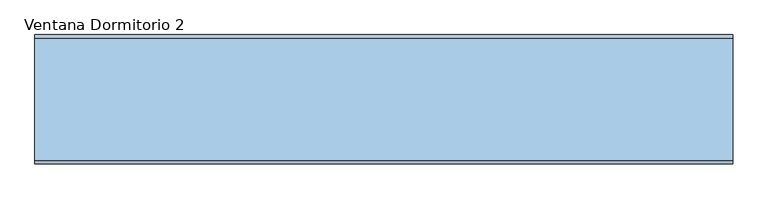
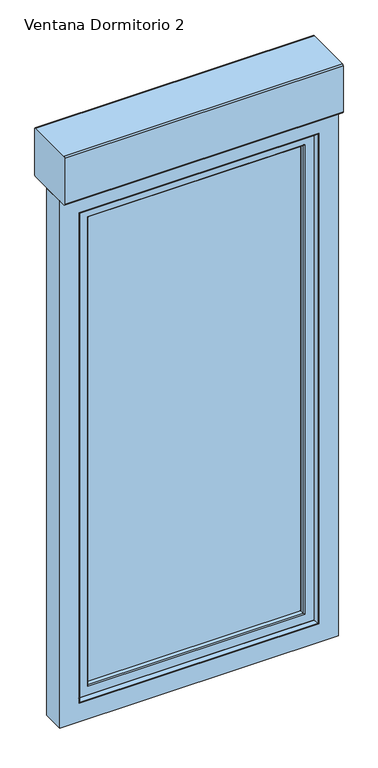
"""IFC4 building model written with IfcOpenShell, lengths in millimetres: window geometry, 2019_ES_Ventana_Replus_re80pvc301_10100_box_1-Hoja_con-Compacto : Ventana Dormitorio 2."""

import ifcopenshell
import ifcopenshell.guid

model = None  # the IFC model being written
_history = None  # IfcOwnerHistory: only IFC2X3 demands one
_inside = {}  # id of a spatial element -> (the spatial element, [elements in it])
_under = {}  # id of a project, library or spatial element -> (it, [spatial elements below it])
_declared = {}  # id of a project -> (the project, [libraries it declares])
_typed = {}  # id of a type object -> (the type object, [elements of that type])
_made_of = {}  # id of a material, layer set ... -> (it, [elements and type objects made of it])


def new_model(schema):
    """Start an empty IFC model of exactly this schema.

    Asked for "IFC4X3", IfcOpenShell would pick the latest addendum, in which some entities
    have other attributes; the version numbers below select the first issue.
    IFC2X3 requires an IfcOwnerHistory on every rooted entity: one is made here for all.
    """
    global model, _history
    if schema == "IFC4X3":
        model = ifcopenshell.file(schema_version=(4, 3, 0, 0))
    else:
        model = ifcopenshell.file(schema=schema)
    _inside.clear()
    _under.clear()
    _declared.clear()
    _typed.clear()
    _made_of.clear()
    _history = None
    if model.schema == "IFC2X3":
        org = make("IfcOrganization", Name="unknown")
        user = make(
            "IfcPersonAndOrganization",
            ThePerson=make("IfcPerson", FamilyName="unknown"),
            TheOrganization=org,
        )
        app = make(
            "IfcApplication",
            ApplicationDeveloper=org,
            Version="unknown",
            ApplicationFullName="unknown",
            ApplicationIdentifier="unknown",
        )
        _history = make(
            "IfcOwnerHistory",
            OwningUser=user,
            OwningApplication=app,
            ChangeAction="ADDED",
            CreationDate=0,
        )
    return model


def make(cls, **values):
    """One entity of the class cls with the attributes given. An attribute that is None is left unset."""
    return model.create_entity(
        cls, **{name: value for name, value in values.items() if value is not None}
    )


def rooted(cls, **values):
    """An entity with a GlobalId (a new one), such as an element, a storey or a relation."""
    return make(cls, GlobalId=ifcopenshell.guid.new(), OwnerHistory=_history, **values)


def si_unit(unit_type, name, prefix=None):
    """IfcSIUnit, for example si_unit("LENGTHUNIT", "METRE", prefix="MILLI")."""
    return make("IfcSIUnit", UnitType=unit_type, Prefix=prefix, Name=name)


def assignment(units):
    """IfcUnitAssignment: the units of a project."""
    return None if units is None else make("IfcUnitAssignment", Units=units)


def point(xyz):
    """IfcCartesianPoint."""
    return None if xyz is None else make("IfcCartesianPoint", Coordinates=xyz)


def direction(xyz):
    """IfcDirection."""
    return None if xyz is None else make("IfcDirection", DirectionRatios=xyz)


def frame(location, z_axis=None, x_axis=None):
    """IfcAxis2Placement3D, a coordinate frame: its origin and axes. An axis left out is left unset."""
    return make(
        "IfcAxis2Placement3D",
        Location=point(location),
        Axis=direction(z_axis),
        RefDirection=direction(x_axis),
    )


def frame_2d(location, x_axis=None):
    """IfcAxis2Placement2D, a coordinate frame in the plane: its origin and x axis."""
    return make(
        "IfcAxis2Placement2D", Location=point(location), RefDirection=direction(x_axis)
    )


def origin():
    """The frame at (0, 0, 0) with its axes left unset."""
    return frame((0.0, 0.0, 0.0))


def place(relative_to, where):
    """IfcLocalPlacement: puts the frame where relative to a parent placement (None: the world)."""
    return make(
        "IfcLocalPlacement", PlacementRelTo=relative_to, RelativePlacement=where
    )


def context(
    kind, dimensions, precision=None, world=None, true_north=None, identifier=None
):
    """IfcGeometricRepresentationContext, for example the 3D "Model" context."""
    return make(
        "IfcGeometricRepresentationContext",
        ContextIdentifier=identifier,
        ContextType=kind,
        CoordinateSpaceDimension=dimensions,
        Precision=precision,
        WorldCoordinateSystem=world,
        TrueNorth=true_north,
    )


def project(units=None, contexts=None):
    """IfcProject with its units and contexts."""
    return rooted(
        "IfcProject",
        Name="project",
        RepresentationContexts=contexts,
        UnitsInContext=assignment(units),
    )


def spatial(cls, under=None, at=None, **own):
    """A site, building, storey or space (cls), placed at a placement, below another one or the project."""
    s = rooted(cls, ObjectPlacement=at, **own)
    if under is not None:
        _under.setdefault(under.id(), (under, []))[1].append(s)
    return s


def polyline(points):
    """IfcPolyline through the points."""
    return make("IfcPolyline", Points=[point(p) for p in points])


def circle_curve(where, radius):
    """IfcCircle in the frame where."""
    return make("IfcCircle", Position=where, Radius=radius)


def ellipse_curve(where, semi_axis1, semi_axis2):
    """IfcEllipse in the frame where."""
    return make(
        "IfcEllipse", Position=where, SemiAxis1=semi_axis1, SemiAxis2=semi_axis2
    )


def trimmed(basis, trim1, trim2, sense, master):
    """IfcTrimmedCurve: the piece of a basis curve between two trims."""
    return make(
        "IfcTrimmedCurve",
        BasisCurve=basis,
        Trim1=trim1,
        Trim2=trim2,
        SenseAgreement=sense,
        MasterRepresentation=master,
    )


def segment(curve, same_sense, transition):
    """IfcCompositeCurveSegment."""
    return make(
        "IfcCompositeCurveSegment",
        Transition=transition,
        SameSense=same_sense,
        ParentCurve=curve,
    )


def composite_curve(segments, self_intersect=None):
    """IfcCompositeCurve: segments joined end to end."""
    return make("IfcCompositeCurve", Segments=segments, SelfIntersect=self_intersect)


def outline(outer, holes=None, kind="AREA"):
    """IfcArbitraryClosedProfileDef: a profile drawn as a closed curve; with holes, ...WithVoids."""
    if holes is None:
        return make("IfcArbitraryClosedProfileDef", ProfileType=kind, OuterCurve=outer)
    return make(
        "IfcArbitraryProfileDefWithVoids",
        ProfileType=kind,
        OuterCurve=outer,
        InnerCurves=holes,
    )


def extrude(swept, where, along, depth):
    """IfcExtrudedAreaSolid: the profile swept, set in the frame where, extruded along a direction by depth."""
    return make(
        "IfcExtrudedAreaSolid",
        SweptArea=swept,
        Position=where,
        ExtrudedDirection=direction(along),
        Depth=depth,
    )


def shape(context_of_items, identifier, shape_type, items):
    """IfcShapeRepresentation: the items that make up one representation, for example the "Body"."""
    return make(
        "IfcShapeRepresentation",
        ContextOfItems=context_of_items,
        RepresentationIdentifier=identifier,
        RepresentationType=shape_type,
        Items=items,
    )


def source(mapping_origin, context_of_items, identifier, shape_type, items):
    """IfcRepresentationMap: a shape defined once, which mapped items show again and again."""
    return make(
        "IfcRepresentationMap",
        MappingOrigin=mapping_origin,
        MappedRepresentation=shape(context_of_items, identifier, shape_type, items),
    )


def transform(
    local_origin,
    x_axis=None,
    y_axis=None,
    z_axis=None,
    scale=None,
    scale2=None,
    scale3=None,
    uniform=True,
):
    """IfcCartesianTransformationOperator3D, or its non-uniform kind. x_axis, y_axis, z_axis: its Axis1, 2, 3."""
    if uniform:
        return make(
            "IfcCartesianTransformationOperator3D",
            Axis1=direction(x_axis),
            Axis2=direction(y_axis),
            LocalOrigin=point(local_origin),
            Scale=scale,
            Axis3=direction(z_axis),
        )
    return make(
        "IfcCartesianTransformationOperator3DnonUniform",
        Axis1=direction(x_axis),
        Axis2=direction(y_axis),
        LocalOrigin=point(local_origin),
        Scale=scale,
        Axis3=direction(z_axis),
        Scale2=scale2,
        Scale3=scale3,
    )


def mapped(mapping_source, mapping_target):
    """IfcMappedItem: shows the shape of a source again, moved by a transform."""
    return make(
        "IfcMappedItem", MappingSource=mapping_source, MappingTarget=mapping_target
    )


def made_of(thing, what):
    """Note that an element or type object is made of a material, layer set ...; save() writes the relation."""
    if what is not None:
        _made_of.setdefault(what.id(), (what, []))[1].append(thing)
    return thing


def element(
    cls,
    number,
    at=None,
    inside=None,
    cuts=None,
    type_object=None,
    material=None,
    context=None,
    identifier="Body",
    shape_type=None,
    held_by="IfcProductDefinitionShape",
    body=None,
    shapes=None,
    **own,
):
    """One element of the class cls, such as IfcWall. Its Tag is "e" and its number.

    at: its placement. inside: the storey or other place that contains it. cuts: it is an
    opening in that element (IfcRelVoidsElement). A single representation is given by context,
    identifier, shape_type and body (its items); several are given by shapes. held_by: the class
    of the entity that holds the representations. save() writes the other relations.
    """
    e = rooted(cls, Tag="e%d" % number, ObjectPlacement=at, **own)
    if body is not None:
        shapes = [shape(context, identifier, shape_type, body)]
    if shapes is not None:
        e.Representation = make(held_by, Representations=shapes)
    if inside is not None:
        _inside.setdefault(inside.id(), (inside, []))[1].append(e)
    if cuts is not None:
        rooted(
            "IfcRelVoidsElement", RelatingBuildingElement=cuts, RelatedOpeningElement=e
        )
    if type_object is not None:
        _typed.setdefault(type_object.id(), (type_object, []))[1].append(e)
    return made_of(e, material)


def aggregate(whole, parts):
    """IfcRelAggregates: a whole, such as a stair, and the parts it consists of."""
    return rooted("IfcRelAggregates", RelatingObject=whole, RelatedObjects=parts)


def save(model, path):
    """Write the relations noted so far, then the file.

    IfcRelAggregates (storeys below a building ...), IfcRelContainedInSpatialStructure (elements
    in a storey), IfcRelDefinesByType, IfcRelAssociatesMaterial and IfcRelDeclares: one each for
    every whole, place, type object, material and project.
    """
    for whole, parts in _under.values():
        aggregate(whole, parts)
    for where, things in _inside.values():
        rooted(
            "IfcRelContainedInSpatialStructure",
            RelatedElements=things,
            RelatingStructure=where,
        )
    for kind, things in _typed.values():
        rooted("IfcRelDefinesByType", RelatedObjects=things, RelatingType=kind)
    for what, things in _made_of.values():
        rooted("IfcRelAssociatesMaterial", RelatedObjects=things, RelatingMaterial=what)
    for by, libraries in _declared.values():
        rooted("IfcRelDeclares", RelatingContext=by, RelatedDefinitions=libraries)
    model.write(path)


def plane_surface(at):
    """IfcPlane: the flat surface through the origin of the frame at, square to its z axis."""
    return make("IfcPlane", Position=at)


def cylinder_surface(at, radius):
    """IfcCylindricalSurface: all points at the distance radius from the z axis of the frame at."""
    return make("IfcCylindricalSurface", Position=at, Radius=radius)


def advanced_brep(points, edges, surfaces, faces):
    """IfcAdvancedBrep: a solid bounded by faces that lie on surfaces and meet in shared edges.

    An edge is (start, end): straight between two places in points (the first is 0);
    or (start, end, curve); or (start, end, curve, False) where it runs against its curve.
    A face is (place in surfaces, loops), or (place, loops, False) where it looks against
    its surface's normal. A loop lists edges by number (the first is 1), with a minus sign
    where the edge is run from its end to its start. The first loop is the outer one.
    """
    corners = [point(p) for p in points]
    vertices = [make("IfcVertexPoint", VertexGeometry=c) for c in corners]
    made = []
    for start, end, *more in edges:
        made.append(
            make(
                "IfcEdgeCurve",
                EdgeStart=vertices[start],
                EdgeEnd=vertices[end],
                EdgeGeometry=more[0] if more else make("IfcPolyline", Points=[corners[start], corners[end]]),
                SameSense=more[1] if len(more) > 1 else True,
            )
        )
    hull = []
    for where, loops, *sense in faces:
        bounds = []
        for j, loop in enumerate(loops):
            ring = [make("IfcOrientedEdge", EdgeElement=made[abs(k) - 1], Orientation=k > 0) for k in loop]
            bounds.append(
                make(
                    "IfcFaceOuterBound" if j == 0 else "IfcFaceBound",
                    Bound=make("IfcEdgeLoop", EdgeList=ring),
                    Orientation=True,
                )
            )
        hull.append(make("IfcAdvancedFace", Bounds=bounds, FaceSurface=surfaces[where], SameSense=sense[0] if sense else True))
    return make("IfcAdvancedBrep", Outer=make("IfcClosedShell", CfsFaces=hull))


def ventana_dormitorio_2_12c73b47(model_context):
    return source(origin(), model_context, "Body", "SolidModel", [
        extrude(outline(composite_curve([segment(trimmed(circle_curve(frame_2d((-55.0, 2815.0)), 5.0), [point((-55.0, 2810.0))], [point((-60.0, 2815.0))], False, "CARTESIAN"), True, "CONTINUOUS"), segment(polyline([(-60.0, 2815.0), (-60.0, 2990.0)]), True, "CONTINUOUS"), segment(trimmed(circle_curve(frame_2d((-55.0, 2990.0)), 5.0), [point((-60.0, 2990.0))], [point((-55.0, 2995.0))], False, "CARTESIAN"), True, "CONTINUOUS"), segment(polyline([(-55.0, 2995.0), (120.0, 2995.0)]), True, "CONTINUOUS"), segment(trimmed(circle_curve(frame_2d((120.0, 2990.0)), 5.0), [point((120.0, 2995.0))], [point((125.0, 2990.0))], False, "CARTESIAN"), True, "CONTINUOUS"), segment(polyline([(125.0, 2990.0), (125.0, 2815.0)]), True, "CONTINUOUS"), segment(trimmed(circle_curve(frame_2d((120.0, 2815.0)), 5.0), [point((125.0, 2815.0))], [point((120.0, 2810.0))], False, "CARTESIAN"), True, "CONTINUOUS"), segment(polyline([(120.0, 2810.0), (-55.0, 2810.0)]), True, "CONTINUOUS")], self_intersect=False)), frame((-500.0, 0.0, 0.0), z_axis=(1.0, 0.0, 0.0), x_axis=(0.0, 1.0, 0.0)), (0.0, 0.0, 1.0), 1000.0),
        extrude(outline(polyline([(78.4999991, 1470.0), (118.4999991, 1470.0), (118.4999991, 1360.0), (98.4999991, 1360.0), (98.4999991, 1450.0), (78.4999991, 1450.0), (78.4999991, 1470.0)])), frame((-434.1999993, 0.0, 0.0), z_axis=(1.0, 0.0, 0.0), x_axis=(0.0, 1.0, 0.0)), (0.0, 0.0, 1.0), 12.0),
        extrude(outline(polyline([(-413.9687607, 78.4999991), (-413.9687607, 68.4999991), (-442.4312378, 68.4999991), (-442.4312378, 78.4999991), (-413.9687607, 78.4999991)])), frame((0.0, 0.0, 1435.217127), z_axis=(0.0, 0.0, 1.0), x_axis=(1.0, 0.0, 0.0)), (0.0, 0.0, 1.0), 49.565746),
        extrude(outline(polyline([(909.8, 397.1999993), (2707.2, 397.1999993), (2707.2, -397.1999993), (909.8, -397.1999993), (909.8, 397.1999993)]), holes=[polyline([(2699.2, 389.1999993), (917.8, 389.1999993), (917.8, -389.1999993), (2699.2, -389.1999993), (2699.2, 389.1999993)])]), frame((0.0, 10.9999999, 0.0), z_axis=(0.0, 1.0, 0.0), x_axis=(0.0, 0.0, 1.0)), (0.0, 0.0, 1.0), 16.0),
        extrude(outline(polyline([(909.8131934, 397.1868058), (2707.1868066, 397.1868058), (2707.1868066, -397.1868058), (909.8131934, -397.1868058), (909.8131934, 397.1868058)]), holes=[polyline([(2699.2, 389.1999993), (917.8, 389.1999993), (917.8, -389.1999993), (2699.2, -389.1999993), (2699.2, 389.1999993)])]), frame((0.0, 31.0000001, 0.0), z_axis=(0.0, 1.0, 0.0), x_axis=(0.0, 0.0, 1.0)), (0.0, 0.0, 1.0), 16.0),
        extrude(outline(polyline([(397.1999993, 6.9999997), (-397.1999993, 6.9999997), (-397.1999993, 10.9999999), (397.1999993, 10.9999999), (397.1999993, 6.9999997)])), frame((0.0, 0.0, 903.7946451), z_axis=(0.0, 0.0, 1.0), x_axis=(1.0, 0.0, 0.0)), (0.0, 0.0, 1.0), 1809.4053549),
        extrude(outline(polyline([(397.1999993, 26.9999999), (-397.1999993, 26.9999999), (-397.1999993, 31.0000001), (397.1999993, 31.0000001), (397.1999993, 26.9999999)])), frame((0.0, 0.0, 903.7946451), z_axis=(0.0, 0.0, 1.0), x_axis=(1.0, 0.0, 0.0)), (0.0, 0.0, 1.0), 1809.4053549),
        extrude(outline(polyline([(397.1999993, 47.0000001), (-397.1999993, 47.0000001), (-397.1999993, 51.0000003), (397.1999993, 51.0000003), (397.1999993, 47.0000001)])), frame((0.0, 0.0, 903.7946451), z_axis=(0.0, 0.0, 1.0), x_axis=(1.0, 0.0, 0.0)), (0.0, 0.0, 1.0), 1809.4053549),
        advanced_brep(
        [(387.2913171, -9.2764571, 2697.2913178), (387.2913171, -9.2764571, 922.7086822), (390.1890946, -11.5, 919.8109047), (390.1890946, -11.5, 2700.1890953), (430.1999993, -11.5, 879.8), (430.1999993, -11.5, 2740.2), (-430.1999993, -11.5, 2740.2), (-430.1999993, -11.5, 879.8), (-390.1890946, -11.5, 919.8109047), (-390.1890946, -11.5, 2700.1890953), (-387.2913171, -9.2764571, 922.7086822), (384.1757968, 2.3508228, 2694.1757976), (384.1757968, 2.3508228, 925.8242024), (-384.1757968, 2.3508228, 925.8242024), (384.6739305, 3.0000033, 2694.6739313), (384.6739305, 3.0000033, 925.3260687), (-384.6739305, 3.0000033, 925.3260687), (391.1999993, 3.0000033, 2701.2), (391.1999993, 3.0000033, 918.8), (-391.1999993, 3.0000033, 918.8), (-391.1999993, 3.0000033, 2701.2), (-384.6739305, 3.0000033, 2694.6739313), (391.1999993, 6.9999997, 2701.2), (391.1999993, 6.9999997, 918.8), (-391.1999993, 6.9999997, 918.8), (411.8162192, 6.9999997, 2721.8162199), (411.8162192, 6.9999997, 898.1837801), (-411.8162192, 6.9999997, 898.1837801), (-411.8162192, 6.9999997, 2721.8162199), (-391.1999993, 6.9999997, 2701.2), (409.1999993, 25.6153717, 2719.2), (409.1999993, 25.6153717, 900.8), (-409.1999993, 25.6153717, 900.8), (409.1999993, 56.4999995, 2719.2), (409.1999993, 56.4999995, 900.8), (-409.1999993, 56.4999995, 900.8), (-409.1999993, 56.4999995, 2719.2), (397.1999993, 56.4999995, 2707.2), (397.1999993, 56.4999995, 912.8), (-397.1999993, 56.4999995, 912.8), (-397.1999993, 56.4999995, 2707.2), (397.1999993, 51.0000003, 2707.2), (397.1999993, 51.0000003, 912.8), (-397.1999993, 51.0000003, 912.8), (-397.1999993, 51.0000003, 2707.2), (386.007687, 51.0000003, 2696.0076877), (386.007687, 51.0000003, 923.9923123), (-386.007687, 51.0000003, 923.9923123), (-386.007687, 51.0000003, 2696.0076877), (385.4940999, 51.6693201, 2695.4941006), (385.4940999, 51.6693201, 924.5058994), (-385.4940999, 51.6693201, 924.5058994), (388.8993918, 64.3780426, 2698.8993925), (388.8993918, 64.3780426, 921.1006075), (-388.8993918, 64.3780426, 921.1006075), (392.6234971, 67.3403297, 2702.6234978), (392.6234971, 67.3403297, 917.3765022), (-392.6234971, 67.3403297, 917.3765022), (405.6488427, 67.7951848, 2715.6488434), (405.6488427, 67.7951848, 904.3511566), (-405.6488427, 67.7951848, 904.3511566), (406.1999993, 67.2629391, 2716.2), (406.1999993, 67.2629391, 903.8), (-406.1999993, 67.2629391, 903.8), (407.4370593, 68.4999991, 2717.43706), (407.4370593, 68.4999991, 902.56294), (-407.4370593, 68.4999991, 902.56294), (460.1999993, 68.4999991, 2770.2), (460.1999993, 68.4999991, 849.8), (-460.1999993, 68.4999991, 849.8), (-460.1999993, 68.4999991, 2770.2), (-407.4370593, 68.4999991, 2717.43706), (463.1999993, 65.4999991, 2773.2), (463.1999993, 65.4999991, 846.8), (-463.1999993, 65.4999991, 846.8), (463.1999993, 50.0, 2773.2), (463.1999993, 50.0, 846.8), (-463.1999993, 50.0, 846.8), (-463.1999993, 50.0, 2773.2), (443.1999993, 50.0, 2753.2), (443.1999993, 50.0, 866.8), (-443.1999993, 50.0, 866.8), (-443.1999993, 50.0, 2753.2), (443.1999993, 11.9999991, 2753.2), (443.1999993, 11.9999991, 866.8), (-443.1999993, 11.9999991, 866.8), (-443.1999993, 11.9999991, 2753.2), (430.1999993, 11.9999991, 2740.2), (430.1999993, 11.9999991, 879.8), (-430.1999993, 11.9999991, 879.8), (-430.1999993, 11.9999991, 2740.2), (-387.2913171, -9.2764571, 2697.2913178), (-384.1757968, 2.3508228, 2694.1757976), (-409.1999993, 25.6153717, 2719.2), (-385.4940999, 51.6693201, 2695.4941006), (-388.8993918, 64.3780426, 2698.8993925), (-392.6234971, 67.3403297, 2702.6234978), (-405.6488427, 67.7951848, 2715.6488434), (-406.1999993, 67.2629391, 2716.2), (-463.1999993, 65.4999991, 2773.2)],
        [
            (0, 1),
            (1, 2, ellipse_curve(frame((390.1890946, -8.5, 919.8109047), z_axis=(0.7071067811865475, 0.0, 0.7071067811865475), x_axis=(-0.7071067811865474, 0.0, 0.7071067811865476)), 4.2426407, 3.0)),
            (2, 3),
            (3, 0, ellipse_curve(frame((390.1890946, -8.5, 2700.1890953), z_axis=(0.7071067811865475, 0.0, -0.7071067811865475), x_axis=(0.7071067811865474, 0.0, 0.7071067811865476)), 4.2426407, 3.0)),
            (4, 5),
            (5, 6),
            (6, 7),
            (7, 4),
            (2, 8),
            (8, 9),
            (9, 3),
            (1, 10),
            (10, 8, ellipse_curve(frame((-390.1890946, -8.5, 919.8109047), z_axis=(0.7071067811865475, 0.0, -0.7071067811865475), x_axis=(0.7071067811865476, 0.0, 0.7071067811865474)), 4.2426407, 3.0)),
            (11, 12),
            (12, 1),
            (0, 11),
            (12, 13),
            (13, 10),
            (14, 15),
            (15, 12, ellipse_curve(frame((384.6739305, 2.4842973, 925.3260687), z_axis=(0.7071067811865475, 0.0, 0.7071067811865475), x_axis=(-0.7071067811865474, 0.0, 0.7071067811865476)), 0.7293184, 0.515706)),
            (11, 14, ellipse_curve(frame((384.6739305, 2.4842973, 2694.6739313), z_axis=(0.7071067811865475, 0.0, -0.7071067811865475), x_axis=(0.7071067811865474, 0.0, 0.7071067811865476)), 0.7293184, 0.515706)),
            (15, 16),
            (16, 13, ellipse_curve(frame((-384.6739305, 2.4842973, 925.3260687), z_axis=(0.7071067811865475, 0.0, -0.7071067811865475), x_axis=(0.7071067811865476, 0.0, 0.7071067811865474)), 0.7293184, 0.515706)),
            (17, 18),
            (18, 19),
            (19, 20),
            (20, 17),
            (14, 21),
            (21, 16),
            (22, 23),
            (23, 18),
            (17, 22),
            (23, 24),
            (24, 19),
            (25, 26),
            (26, 27),
            (27, 28),
            (28, 25),
            (22, 29),
            (29, 24),
            (30, 31),
            (31, 26),
            (25, 30),
            (31, 32),
            (32, 27),
            (33, 34),
            (34, 31),
            (30, 33),
            (34, 35),
            (35, 32),
            (33, 36),
            (36, 35),
            (37, 38),
            (38, 39),
            (39, 40),
            (40, 37),
            (41, 42),
            (42, 38),
            (37, 41),
            (42, 43),
            (43, 39),
            (41, 44),
            (44, 43),
            (45, 46),
            (46, 47),
            (47, 48),
            (48, 45),
            (49, 50),
            (50, 46, ellipse_curve(frame((386.007687, 51.5317048, 923.9923123), z_axis=(0.7071067811865475, 0.0, 0.7071067811865475), x_axis=(-0.7071067811865474, 0.0, 0.7071067811865476)), 0.7519437, 0.5317045)),
            (45, 49, ellipse_curve(frame((386.007687, 51.5317048, 2696.0076877), z_axis=(0.7071067811865475, 0.0, -0.7071067811865475), x_axis=(0.7071067811865474, 0.0, 0.7071067811865476)), 0.7519437, 0.5317045)),
            (50, 51),
            (51, 47, ellipse_curve(frame((-386.007687, 51.5317048, 923.9923123), z_axis=(0.7071067811865475, 0.0, -0.7071067811865475), x_axis=(0.7071067811865476, 0.0, 0.7071067811865474)), 0.7519437, 0.5317045)),
            (52, 53),
            (53, 50),
            (49, 52),
            (53, 54),
            (54, 51),
            (55, 56),
            (56, 53, ellipse_curve(frame((392.7630951, 63.3427664, 917.2369042), z_axis=(0.7071067811865475, 0.0, 0.7071067811865475), x_axis=(-0.7071067811865474, 0.0, 0.7071067811865476)), 5.6568542, 4.0)),
            (52, 55, ellipse_curve(frame((392.7630951, 63.3427664, 2702.7630958), z_axis=(0.7071067811865475, 0.0, -0.7071067811865475), x_axis=(0.7071067811865474, 0.0, 0.7071067811865476)), 5.6568542, 4.0)),
            (56, 57),
            (57, 54, ellipse_curve(frame((-392.7630951, 63.3427664, 917.2369042), z_axis=(0.7071067811865475, 0.0, -0.7071067811865475), x_axis=(0.7071067811865476, 0.0, 0.7071067811865474)), 5.6568542, 4.0)),
            (58, 59),
            (59, 56),
            (55, 58),
            (59, 60),
            (60, 57),
            (61, 62),
            (62, 59, ellipse_curve(frame((405.6674291, 67.2629391, 904.3325701), z_axis=(0.7071067811865475, 0.0, 0.7071067811865475), x_axis=(-0.7071067811865474, 0.0, 0.7071067811865476)), 0.7531679, 0.5325701)),
            (58, 61, ellipse_curve(frame((405.6674291, 67.2629391, 2715.6674299), z_axis=(0.7071067811865475, 0.0, -0.7071067811865475), x_axis=(0.7071067811865474, 0.0, 0.7071067811865476)), 0.7531679, 0.5325701)),
            (62, 63),
            (63, 60, ellipse_curve(frame((-405.6674291, 67.2629391, 904.3325701), z_axis=(0.7071067811865475, 0.0, -0.7071067811865475), x_axis=(0.7071067811865476, 0.0, 0.7071067811865474)), 0.7531679, 0.5325701)),
            (64, 65),
            (65, 62, ellipse_curve(frame((407.4370593, 67.2629391, 902.56294), z_axis=(0.7071067811865475, 0.0, 0.7071067811865475), x_axis=(-0.7071067811865474, 0.0, 0.7071067811865476)), 1.7494671, 1.23706)),
            (61, 64, ellipse_curve(frame((407.4370593, 67.2629391, 2717.43706), z_axis=(0.7071067811865475, 0.0, -0.7071067811865475), x_axis=(0.7071067811865474, 0.0, 0.7071067811865476)), 1.7494671, 1.23706)),
            (65, 66),
            (66, 63, ellipse_curve(frame((-407.4370593, 67.2629391, 902.56294), z_axis=(0.7071067811865475, 0.0, -0.7071067811865475), x_axis=(0.7071067811865476, 0.0, 0.7071067811865474)), 1.7494671, 1.23706)),
            (67, 68),
            (68, 69),
            (69, 70),
            (70, 67),
            (64, 71),
            (71, 66),
            (72, 73),
            (73, 68, ellipse_curve(frame((460.1999993, 65.4999991, 849.8), z_axis=(0.7071067811865475, 0.0, 0.7071067811865475), x_axis=(-0.7071067811865474, 0.0, 0.7071067811865476)), 4.2426407, 3.0)),
            (67, 72, ellipse_curve(frame((460.1999993, 65.4999991, 2770.2), z_axis=(0.7071067811865475, 0.0, -0.7071067811865475), x_axis=(0.7071067811865474, 0.0, 0.7071067811865476)), 4.2426407, 3.0)),
            (73, 74),
            (74, 69, ellipse_curve(frame((-460.1999993, 65.4999991, 849.8), z_axis=(0.7071067811865475, 0.0, -0.7071067811865475), x_axis=(0.7071067811865476, 0.0, 0.7071067811865474)), 4.2426407, 3.0)),
            (75, 76),
            (76, 73),
            (72, 75),
            (76, 77),
            (77, 74),
            (75, 78),
            (78, 77),
            (79, 80),
            (80, 81),
            (81, 82),
            (82, 79),
            (79, 83),
            (83, 84),
            (84, 80),
            (84, 85),
            (85, 81),
            (83, 86),
            (86, 85),
            (87, 88),
            (88, 89),
            (89, 90),
            (90, 87),
            (87, 5),
            (4, 88),
            (7, 89),
            (10, 91),
            (91, 9, ellipse_curve(frame((-390.1890946, -8.5, 2700.1890953), z_axis=(-0.7071067811865475, 0.0, -0.7071067811865475), x_axis=(0.7071067811865474, 0.0, -0.7071067811865476)), 4.2426407, 3.0)),
            (13, 92),
            (92, 91),
            (21, 92, ellipse_curve(frame((-384.6739305, 2.4842973, 2694.6739313), z_axis=(-0.7071067811865475, 0.0, -0.7071067811865475), x_axis=(0.7071067811865474, 0.0, -0.7071067811865476)), 0.7293184, 0.515706)),
            (29, 20),
            (32, 93),
            (93, 28),
            (36, 93),
            (44, 40),
            (51, 94),
            (94, 48, ellipse_curve(frame((-386.007687, 51.5317048, 2696.0076877), z_axis=(-0.7071067811865475, 0.0, -0.7071067811865475), x_axis=(0.7071067811865474, 0.0, -0.7071067811865476)), 0.7519437, 0.5317045)),
            (54, 95),
            (95, 94),
            (57, 96),
            (96, 95, ellipse_curve(frame((-392.7630951, 63.3427664, 2702.7630958), z_axis=(-0.7071067811865475, 0.0, -0.7071067811865475), x_axis=(0.7071067811865474, 0.0, -0.7071067811865476)), 5.6568542, 4.0)),
            (60, 97),
            (97, 96),
            (63, 98),
            (98, 97, ellipse_curve(frame((-405.6674291, 67.2629391, 2715.6674299), z_axis=(-0.7071067811865475, 0.0, -0.7071067811865475), x_axis=(0.7071067811865474, 0.0, -0.7071067811865476)), 0.7531679, 0.5325701)),
            (71, 98, ellipse_curve(frame((-407.4370593, 67.2629391, 2717.43706), z_axis=(-0.7071067811865475, 0.0, -0.7071067811865475), x_axis=(0.7071067811865474, 0.0, -0.7071067811865476)), 1.7494671, 1.23706)),
            (74, 99),
            (99, 70, ellipse_curve(frame((-460.1999993, 65.4999991, 2770.2), z_axis=(-0.7071067811865475, 0.0, -0.7071067811865475), x_axis=(0.7071067811865474, 0.0, -0.7071067811865476)), 4.2426407, 3.0)),
            (78, 99),
            (86, 82),
            (6, 90),
            (91, 0),
            (92, 11),
            (93, 30),
            (94, 49),
            (95, 52),
            (96, 55),
            (97, 58),
            (98, 61),
            (99, 72),
        ],
        [
            cylinder_surface(frame((390.1890946, -8.5, 2773.2), z_axis=(0.0, 0.0, 1.0), x_axis=(-1.0, 0.0, 0.0)), 3.0),
            plane_surface(frame((-430.1999993, -11.5, 2740.2), z_axis=(0.0, -1.0, 0.0), x_axis=(1.0, 0.0, 0.0))),
            cylinder_surface(frame((463.1999993, -8.5, 919.8109047), z_axis=(1.0, 0.0, 0.0), x_axis=(0.0, 0.0, 1.0)), 3.0),
            plane_surface(frame((387.2913171, -9.2764571, 2697.2913178), z_axis=(-0.9659258263570549, -0.2588190448487916, 0.0), x_axis=(0.0, 0.0, -1.0))),
            plane_surface(frame((387.2913171, -9.2764571, 922.7086822), z_axis=(0.0, -0.2588190448487885, 0.9659258263570558), x_axis=(-1.0, 0.0, 0.0))),
            cylinder_surface(frame((384.6739305, 2.4842973, 2773.2), z_axis=(0.0, 0.0, 1.0), x_axis=(-1.0, 0.0, 0.0)), 0.515706),
            cylinder_surface(frame((463.1999993, 2.4842973, 925.3260687), z_axis=(1.0, 0.0, 0.0), x_axis=(0.0, 0.0, 1.0)), 0.515706),
            plane_surface(frame((-384.6739305, 3.0000033, 2694.6739313), z_axis=(0.0, 1.0, 0.0), x_axis=(1.0, 0.0, 0.0))),
            plane_surface(frame((391.1999993, 3.0000033, 2701.2), z_axis=(-1.0, 0.0, 0.0), x_axis=(0.0, 0.0, -1.0))),
            plane_surface(frame((391.1999993, 3.0000033, 918.8), z_axis=(0.0, 0.0, 1.0), x_axis=(-1.0, 0.0, 0.0))),
            plane_surface(frame((-391.1999993, 6.9999997, 2701.2), z_axis=(0.0, 1.0, 0.0), x_axis=(1.0, 0.0, 0.0))),
            plane_surface(frame((411.8162192, 6.9999997, 2721.8162199), z_axis=(-0.9902680687415736, -0.13917310096004265, 0.0), x_axis=(0.0, 0.0, -1.0))),
            plane_surface(frame((411.8162192, 6.9999997, 898.1837801), z_axis=(0.0, -0.13917310096003946, 0.990268068741574), x_axis=(-1.0, 0.0, 0.0))),
            plane_surface(frame((409.1999993, 25.6153717, 2719.2), z_axis=(-1.0, 0.0, 0.0), x_axis=(0.0, 0.0, -1.0))),
            plane_surface(frame((409.1999993, 25.6153717, 900.8), z_axis=(0.0, 0.0, 1.0), x_axis=(-1.0, 0.0, 0.0))),
            plane_surface(frame((-409.1999993, 56.4999995, 2719.2), z_axis=(0.0, -1.0, 0.0), x_axis=(1.0, 0.0, 0.0))),
            plane_surface(frame((397.1999993, 56.4999995, 2707.2), z_axis=(1.0, 0.0, 0.0), x_axis=(0.0, 0.0, -1.0))),
            plane_surface(frame((397.1999993, 56.4999995, 912.8), z_axis=(0.0, 0.0, -1.0), x_axis=(-1.0, 0.0, 0.0))),
            plane_surface(frame((-397.1999993, 51.0000003, 2707.2), z_axis=(0.0, -1.0, 0.0), x_axis=(1.0, 0.0, 0.0))),
            cylinder_surface(frame((386.007687, 51.5317048, 2773.2), z_axis=(0.0, 0.0, 1.0), x_axis=(-1.0, 0.0, 0.0)), 0.5317045),
            cylinder_surface(frame((463.1999993, 51.5317048, 923.9923123), z_axis=(1.0, 0.0, 0.0), x_axis=(0.0, 0.0, 1.0)), 0.5317045),
            plane_surface(frame((385.4940999, 51.6693201, 2695.4941006), z_axis=(-0.9659258262890666, 0.2588190451025272, 0.0), x_axis=(0.0, 0.0, -1.0))),
            plane_surface(frame((385.4940999, 51.6693201, 924.5058994), z_axis=(0.0, 0.2588190451025303, 0.9659258262890658), x_axis=(-1.0, 0.0, 0.0))),
            cylinder_surface(frame((392.7630951, 63.3427664, 2773.2), z_axis=(0.0, 0.0, 1.0), x_axis=(-1.0, 0.0, 0.0)), 4.0),
            cylinder_surface(frame((463.1999993, 63.3427664, 917.2369042), z_axis=(1.0, 0.0, 0.0), x_axis=(0.0, 0.0, 1.0)), 4.0),
            plane_surface(frame((392.6234971, 67.3403297, 2702.6234978), z_axis=(-0.034899496702507804, 0.9993908270190955, 0.0), x_axis=(0.0, 0.0, -1.0))),
            plane_surface(frame((392.6234971, 67.3403297, 917.3765022), z_axis=(0.0, 0.9993908270190957, 0.03489949670250457), x_axis=(-1.0, 0.0, 0.0))),
            cylinder_surface(frame((405.6674291, 67.2629391, 2773.2), z_axis=(0.0, 0.0, 1.0), x_axis=(-1.0, 0.0, 0.0)), 0.5325701),
            cylinder_surface(frame((463.1999993, 67.2629391, 904.3325701), z_axis=(1.0, 0.0, 0.0), x_axis=(0.0, 0.0, 1.0)), 0.5325701),
            cylinder_surface(frame((407.4370593, 67.2629391, 2773.2), z_axis=(0.0, 0.0, 1.0), x_axis=(-1.0, 0.0, 0.0)), 1.23706),
            cylinder_surface(frame((463.1999993, 67.2629391, 902.56294), z_axis=(1.0, 0.0, 0.0), x_axis=(0.0, 0.0, 1.0)), 1.23706),
            plane_surface(frame((-407.4370593, 68.4999991, 2717.43706), z_axis=(0.0, 1.0, 0.0), x_axis=(1.0, 0.0, 0.0))),
            cylinder_surface(frame((460.1999993, 65.4999991, 2773.2), z_axis=(0.0, 0.0, 1.0), x_axis=(-1.0, 0.0, 0.0)), 3.0),
            cylinder_surface(frame((463.1999993, 65.4999991, 849.8), z_axis=(1.0, 0.0, 0.0), x_axis=(0.0, 0.0, 1.0)), 3.0),
            plane_surface(frame((463.1999993, 65.4999991, 2773.2), z_axis=(1.0, 0.0, 0.0), x_axis=(0.0, 0.0, -1.0))),
            plane_surface(frame((463.1999993, 65.4999991, 846.8), z_axis=(0.0, 0.0, -1.0), x_axis=(-1.0, 0.0, 0.0))),
            plane_surface(frame((-459.2000019, 50.0, 2769.2000027), z_axis=(0.0, -1.0, 0.0), x_axis=(1.0, 0.0, 0.0))),
            plane_surface(frame((443.1999993, 45.0999991, 2753.2), z_axis=(1.0, 0.0, 0.0), x_axis=(0.0, 0.0, -1.0))),
            plane_surface(frame((443.1999993, 45.0999991, 866.8), z_axis=(0.0, 0.0, -1.0), x_axis=(-1.0, 0.0, 0.0))),
            plane_surface(frame((-435.7000002, 11.9999991, 2745.7000009), z_axis=(0.0, -1.0, 0.0), x_axis=(1.0, 0.0, 0.0))),
            plane_surface(frame((430.1999993, 1.4999991, 2740.2), z_axis=(1.0, 0.0, 0.0), x_axis=(0.0, 0.0, -1.0))),
            plane_surface(frame((430.1999993, 1.4999991, 879.8), z_axis=(0.0, 0.0, -1.0), x_axis=(-1.0, 0.0, 0.0))),
            cylinder_surface(frame((-390.1890946, -8.5, 846.8), z_axis=(0.0, 0.0, -1.0), x_axis=(1.0, 0.0, 0.0)), 3.0),
            plane_surface(frame((-387.2913171, -9.2764571, 922.7086822), z_axis=(0.9659258263570565, -0.2588190448487853, 0.0), x_axis=(0.0, 0.0, 1.0))),
            cylinder_surface(frame((-384.6739305, 2.4842973, 846.8), z_axis=(0.0, 0.0, -1.0), x_axis=(1.0, 0.0, 0.0)), 0.515706),
            plane_surface(frame((-391.1999993, 3.0000033, 918.8), z_axis=(1.0, 0.0, 0.0), x_axis=(0.0, 0.0, 1.0))),
            plane_surface(frame((-411.8162192, 6.9999997, 898.1837801), z_axis=(0.9902680687415745, -0.13917310096003627, 0.0), x_axis=(0.0, 0.0, 1.0))),
            plane_surface(frame((-409.1999993, 25.6153717, 900.8), z_axis=(1.0, 0.0, 0.0), x_axis=(0.0, 0.0, 1.0))),
            plane_surface(frame((-397.1999993, 56.4999995, 912.8), z_axis=(-1.0, 0.0, 0.0), x_axis=(0.0, 0.0, 1.0))),
            cylinder_surface(frame((-386.007687, 51.5317048, 846.8), z_axis=(0.0, 0.0, -1.0), x_axis=(1.0, 0.0, 0.0)), 0.5317045),
            plane_surface(frame((-385.4940999, 51.6693201, 924.5058994), z_axis=(0.9659258262890649, 0.2588190451025334, 0.0), x_axis=(0.0, 0.0, 1.0))),
            cylinder_surface(frame((-392.7630951, 63.3427664, 846.8), z_axis=(0.0, 0.0, -1.0), x_axis=(1.0, 0.0, 0.0)), 4.0),
            plane_surface(frame((-392.6234971, 67.3403297, 917.3765022), z_axis=(0.03489949670250134, 0.9993908270190958, 0.0), x_axis=(0.0, 0.0, 1.0))),
            cylinder_surface(frame((-405.6674291, 67.2629391, 846.8), z_axis=(0.0, 0.0, -1.0), x_axis=(1.0, 0.0, 0.0)), 0.5325701),
            cylinder_surface(frame((-407.4370593, 67.2629391, 846.8), z_axis=(0.0, 0.0, -1.0), x_axis=(1.0, 0.0, 0.0)), 1.23706),
            cylinder_surface(frame((-460.1999993, 65.4999991, 846.8), z_axis=(0.0, 0.0, -1.0), x_axis=(1.0, 0.0, 0.0)), 3.0),
            plane_surface(frame((-463.1999993, 65.4999991, 846.8), z_axis=(-1.0, 0.0, 0.0), x_axis=(0.0, 0.0, 1.0))),
            plane_surface(frame((-443.1999993, 45.0999991, 866.8), z_axis=(-1.0, 0.0, 0.0), x_axis=(0.0, 0.0, 1.0))),
            plane_surface(frame((-430.1999993, 1.4999991, 879.8), z_axis=(-1.0, 0.0, 0.0), x_axis=(0.0, 0.0, 1.0))),
            cylinder_surface(frame((-463.1999993, -8.5, 2700.1890953), z_axis=(-1.0, 0.0, 0.0), x_axis=(0.0, 0.0, -1.0)), 3.0),
            plane_surface(frame((-387.2913171, -9.2764571, 2697.2913178), z_axis=(0.0, -0.2588190448487885, -0.9659258263570557), x_axis=(1.0, 0.0, 0.0))),
            cylinder_surface(frame((-463.1999993, 2.4842973, 2694.6739313), z_axis=(-1.0, 0.0, 0.0), x_axis=(0.0, 0.0, -1.0)), 0.515706),
            plane_surface(frame((-391.1999993, 3.0000033, 2701.2), z_axis=(0.0, 0.0, -1.0), x_axis=(1.0, 0.0, 0.0))),
            plane_surface(frame((-411.8162192, 6.9999997, 2721.8162199), z_axis=(0.0, -0.13917310096003946, -0.990268068741574), x_axis=(1.0, 0.0, 0.0))),
            plane_surface(frame((-409.1999993, 25.6153717, 2719.2), z_axis=(0.0, 0.0, -1.0), x_axis=(1.0, 0.0, 0.0))),
            plane_surface(frame((-397.1999993, 56.4999995, 2707.2), z_axis=(0.0, 0.0, 1.0), x_axis=(1.0, 0.0, 0.0))),
            cylinder_surface(frame((-463.1999993, 51.5317048, 2696.0076877), z_axis=(-1.0, 0.0, 0.0), x_axis=(0.0, 0.0, -1.0)), 0.5317045),
            plane_surface(frame((-385.4940999, 51.6693201, 2695.4941006), z_axis=(0.0, 0.2588190451025303, -0.9659258262890658), x_axis=(1.0, 0.0, 0.0))),
            cylinder_surface(frame((-463.1999993, 63.3427664, 2702.7630958), z_axis=(-1.0, 0.0, 0.0), x_axis=(0.0, 0.0, -1.0)), 4.0),
            plane_surface(frame((-392.6234971, 67.3403297, 2702.6234978), z_axis=(0.0, 0.9993908270190957, -0.03489949670250457), x_axis=(1.0, 0.0, 0.0))),
            cylinder_surface(frame((-463.1999993, 67.2629391, 2715.6674299), z_axis=(-1.0, 0.0, 0.0), x_axis=(0.0, 0.0, -1.0)), 0.5325701),
            cylinder_surface(frame((-463.1999993, 67.2629391, 2717.43706), z_axis=(-1.0, 0.0, 0.0), x_axis=(0.0, 0.0, -1.0)), 1.23706),
            cylinder_surface(frame((-463.1999993, 65.4999991, 2770.2), z_axis=(-1.0, 0.0, 0.0), x_axis=(0.0, 0.0, -1.0)), 3.0),
            plane_surface(frame((-463.1999993, 65.4999991, 2773.2), z_axis=(0.0, 0.0, 1.0), x_axis=(1.0, 0.0, 0.0))),
            plane_surface(frame((-443.1999993, 45.0999991, 2753.2), z_axis=(0.0, 0.0, 1.0), x_axis=(1.0, 0.0, 0.0))),
            plane_surface(frame((-430.1999993, 1.4999991, 2740.2), z_axis=(0.0, 0.0, 1.0), x_axis=(1.0, 0.0, 0.0))),
        ],
        [
            (0, [[1, 2, 3, 4]]),
            (1, [[5, 6, 7, 8], [-3, 9, 10, 11]]),
            (2, [[12, 13, -9, -2]]),
            (3, [[14, 15, -1, 16]]),
            (4, [[17, 18, -12, -15]]),
            (5, [[19, 20, -14, 21]]),
            (6, [[22, 23, -17, -20]]),
            (7, [[24, 25, 26, 27], [-19, 28, 29, -22]]),
            (8, [[30, 31, -24, 32]]),
            (9, [[33, 34, -25, -31]]),
            (10, [[35, 36, 37, 38], [-30, 39, 40, -33]]),
            (11, [[41, 42, -35, 43]]),
            (12, [[44, 45, -36, -42]]),
            (13, [[46, 47, -41, 48]]),
            (14, [[49, 50, -44, -47]]),
            (15, [[-46, 51, 52, -49], [53, 54, 55, 56]]),
            (16, [[57, 58, -53, 59]]),
            (17, [[60, 61, -54, -58]]),
            (18, [[-57, 62, 63, -60], [64, 65, 66, 67]]),
            (19, [[68, 69, -64, 70]]),
            (20, [[71, 72, -65, -69]]),
            (21, [[73, 74, -68, 75]]),
            (22, [[76, 77, -71, -74]]),
            (23, [[78, 79, -73, 80]]),
            (24, [[81, 82, -76, -79]]),
            (25, [[83, 84, -78, 85]]),
            (26, [[86, 87, -81, -84]]),
            (27, [[88, 89, -83, 90]]),
            (28, [[91, 92, -86, -89]]),
            (29, [[93, 94, -88, 95]]),
            (30, [[96, 97, -91, -94]]),
            (31, [[98, 99, 100, 101], [-93, 102, 103, -96]]),
            (32, [[104, 105, -98, 106]]),
            (33, [[107, 108, -99, -105]]),
            (34, [[109, 110, -104, 111]]),
            (35, [[112, 113, -107, -110]]),
            (36, [[-109, 114, 115, -112], [116, 117, 118, 119]]),
            (37, [[120, 121, 122, -116]]),
            (38, [[123, 124, -117, -122]]),
            (39, [[-121, 125, 126, -123], [127, 128, 129, 130]]),
            (40, [[131, -5, 132, -127]]),
            (41, [[-8, 133, -128, -132]]),
            (42, [[134, 135, -10, -13]]),
            (43, [[136, 137, -134, -18]]),
            (44, [[-29, 138, -136, -23]]),
            (45, [[-40, 139, -26, -34]]),
            (46, [[140, 141, -37, -45]]),
            (47, [[-52, 142, -140, -50]]),
            (48, [[-63, 143, -55, -61]]),
            (49, [[144, 145, -66, -72]]),
            (50, [[146, 147, -144, -77]]),
            (51, [[148, 149, -146, -82]]),
            (52, [[150, 151, -148, -87]]),
            (53, [[152, 153, -150, -92]]),
            (54, [[-103, 154, -152, -97]]),
            (55, [[155, 156, -100, -108]]),
            (56, [[-115, 157, -155, -113]]),
            (57, [[-126, 158, -118, -124]]),
            (58, [[-7, 159, -129, -133]]),
            (59, [[160, -4, -11, -135]]),
            (60, [[161, -16, -160, -137]]),
            (61, [[-28, -21, -161, -138]]),
            (62, [[-39, -32, -27, -139]]),
            (63, [[162, -43, -38, -141]]),
            (64, [[-51, -48, -162, -142]]),
            (65, [[-62, -59, -56, -143]]),
            (66, [[163, -70, -67, -145]]),
            (67, [[164, -75, -163, -147]]),
            (68, [[165, -80, -164, -149]]),
            (69, [[166, -85, -165, -151]]),
            (70, [[167, -90, -166, -153]]),
            (71, [[-102, -95, -167, -154]]),
            (72, [[168, -106, -101, -156]]),
            (73, [[-114, -111, -168, -157]]),
            (74, [[-125, -120, -119, -158]]),
            (75, [[-6, -131, -130, -159]]),
        ],
    ),
        advanced_brep(
        [(423.2673545, -12.758819, 2733.2673545), (423.2673545, -12.758819, 886.7326455), (427.2913185, -27.7764571, 882.7086815), (427.2913185, -27.7764571, 2737.2913185), (430.189096, -30.0, 879.810904), (430.189096, -30.0, 2740.189096), (-423.2673545, -12.758819, 886.7326455), (-427.2913185, -27.7764571, 882.7086815), (424.2332803, -11.5, 2734.2332803), (424.2332803, -11.5, 885.7667197), (500.0, -30.0, 2810.0), (500.0, -30.0, 810.0), (500.0, 50.0, 810.0), (500.0, 50.0, 2810.0), (-500.0, 50.0, 810.0), (-500.0, 50.0, 2810.0), (456.1999993, 50.0, 853.8000007), (456.1999993, 50.0, 2766.1999993), (-456.1999993, 50.0, 2766.1999993), (-456.1999993, 50.0, 853.8000007), (-500.0, -30.0, 810.0), (-500.0, -30.0, 2810.0), (-430.189096, -30.0, 879.810904), (-430.189096, -30.0, 2740.189096), (436.1891471, 8.0, 2746.1891471), (436.1891471, 8.0, 873.8108529), (436.1891471, -11.5, 873.8108529), (436.1891471, -11.5, 2746.1891471), (-436.1891471, -11.5, 873.8108529), (-436.1891471, -11.5, 2746.1891471), (-424.2332803, -11.5, 2734.2332803), (-424.2332803, -11.5, 885.7667197), (-436.1891471, 8.0, 873.8108529), (455.1999993, 8.0, 2765.1999993), (455.1999993, 8.0, 854.8000007), (-455.1999993, 8.0, 854.8000007), (-455.1999993, 8.0, 2765.1999993), (-436.1891471, 8.0, 2746.1891471), (455.1999993, 49.0, 854.8000007), (455.1999993, 49.0, 2765.1999993), (-455.1999993, 49.0, 854.8000007), (-423.2673545, -12.758819, 2733.2673545), (-427.2913185, -27.7764571, 2737.2913185), (-455.1999993, 49.0, 2765.1999993)],
        [
            (0, 1),
            (1, 2),
            (2, 3),
            (3, 0),
            (2, 4, ellipse_curve(frame((430.189096, -27.0, 879.810904), z_axis=(0.7071067811865475, 0.0, 0.7071067811865475), x_axis=(-0.7071067811865474, 0.0, 0.7071067811865476)), 4.2426407, 3.0)),
            (4, 5),
            (5, 3, ellipse_curve(frame((430.189096, -27.0, 2740.189096), z_axis=(0.7071067811865475, 0.0, -0.7071067811865475), x_axis=(0.7071067811865474, 0.0, 0.7071067811865476)), 4.2426407, 3.0)),
            (1, 6),
            (6, 7),
            (7, 2),
            (8, 9),
            (9, 1, ellipse_curve(frame((424.2332803, -12.5, 885.7667197), z_axis=(0.7071067811865475, 0.0, 0.7071067811865475), x_axis=(-0.7071067811865474, 0.0, 0.7071067811865476)), 1.4142136, 1.0)),
            (0, 8, ellipse_curve(frame((424.2332803, -12.5, 2734.2332803), z_axis=(0.7071067811865475, 0.0, -0.7071067811865475), x_axis=(0.7071067811865474, 0.0, 0.7071067811865476)), 1.4142136, 1.0)),
            (10, 11),
            (11, 12),
            (12, 13),
            (13, 10),
            (12, 14),
            (14, 15),
            (15, 13),
            (16, 17),
            (17, 18),
            (18, 19),
            (19, 16),
            (11, 20),
            (20, 14),
            (10, 21),
            (21, 20),
            (4, 22),
            (22, 23),
            (23, 5),
            (24, 25),
            (25, 26),
            (26, 27),
            (27, 24),
            (26, 28),
            (28, 29),
            (29, 27),
            (8, 30),
            (30, 31),
            (31, 9),
            (25, 32),
            (32, 28),
            (33, 34),
            (34, 35),
            (35, 36),
            (36, 33),
            (24, 37),
            (37, 32),
            (16, 38, ellipse_curve(frame((456.1999993, 49.0, 853.8000007), z_axis=(0.7071067811865475, 0.0, 0.7071067811865475), x_axis=(-0.7071067811865474, 0.0, 0.7071067811865476)), 1.4142136, 1.0)),
            (38, 39),
            (39, 17, ellipse_curve(frame((456.1999993, 49.0, 2766.1999993), z_axis=(0.7071067811865475, 0.0, -0.7071067811865475), x_axis=(0.7071067811865474, 0.0, 0.7071067811865476)), 1.4142136, 1.0)),
            (38, 34),
            (33, 39),
            (19, 40, ellipse_curve(frame((-456.1999993, 49.0, 853.8000007), z_axis=(0.7071067811865475, 0.0, -0.7071067811865475), x_axis=(0.7071067811865476, 0.0, 0.7071067811865474)), 1.4142136, 1.0)),
            (40, 38),
            (31, 6, ellipse_curve(frame((-424.2332803, -12.5, 885.7667197), z_axis=(0.7071067811865475, 0.0, -0.7071067811865475), x_axis=(0.7071067811865476, 0.0, 0.7071067811865474)), 1.4142136, 1.0)),
            (7, 22, ellipse_curve(frame((-430.189096, -27.0, 879.810904), z_axis=(0.7071067811865475, 0.0, -0.7071067811865475), x_axis=(0.7071067811865476, 0.0, 0.7071067811865474)), 4.2426407, 3.0)),
            (6, 41),
            (41, 42),
            (42, 7),
            (21, 15),
            (37, 29),
            (40, 35),
            (18, 43, ellipse_curve(frame((-456.1999993, 49.0, 2766.1999993), z_axis=(-0.7071067811865475, 0.0, -0.7071067811865475), x_axis=(0.7071067811865474, 0.0, -0.7071067811865476)), 1.4142136, 1.0)),
            (43, 40),
            (30, 41, ellipse_curve(frame((-424.2332803, -12.5, 2734.2332803), z_axis=(-0.7071067811865475, 0.0, -0.7071067811865475), x_axis=(0.7071067811865474, 0.0, -0.7071067811865476)), 1.4142136, 1.0)),
            (42, 23, ellipse_curve(frame((-430.189096, -27.0, 2740.189096), z_axis=(-0.7071067811865475, 0.0, -0.7071067811865475), x_axis=(0.7071067811865474, 0.0, -0.7071067811865476)), 4.2426407, 3.0)),
            (43, 36),
            (41, 0),
            (3, 42),
            (39, 43),
        ],
        [
            plane_surface(frame((427.2913185, -27.7764571, 2737.2913185), z_axis=(-0.9659258262890693, -0.2588190451025169, 0.0), x_axis=(0.0, 0.0, -1.0))),
            cylinder_surface(frame((430.189096, -27.0, 2810.0), z_axis=(0.0, 0.0, 1.0), x_axis=(-1.0, 0.0, 0.0)), 3.0),
            plane_surface(frame((427.2913185, -27.7764571, 882.7086815), z_axis=(0.0, -0.2588190451025138, 0.9659258262890702), x_axis=(-1.0, 0.0, 0.0))),
            cylinder_surface(frame((424.2332803, -12.5, 2810.0), z_axis=(0.0, 0.0, 1.0), x_axis=(-1.0, 0.0, 0.0)), 1.0),
            plane_surface(frame((500.0, 50.0, 2810.0), z_axis=(1.0, 0.0, 0.0), x_axis=(0.0, 0.0, -1.0))),
            plane_surface(frame((-456.1999993, 50.0, 2766.1999993), z_axis=(0.0, 1.0, 0.0), x_axis=(1.0, 0.0, 0.0))),
            plane_surface(frame((500.0, 50.0, 810.0), z_axis=(0.0, 0.0, -1.0), x_axis=(-1.0, 0.0, 0.0))),
            plane_surface(frame((-500.0, -30.0, 2810.0), z_axis=(0.0, -1.0, 0.0), x_axis=(1.0, 0.0, 0.0))),
            plane_surface(frame((436.1891471, -11.5, 2746.1891471), z_axis=(-1.0, 0.0, 0.0), x_axis=(0.0, 0.0, -1.0))),
            plane_surface(frame((-424.2332803, -11.5, 2734.2332803), z_axis=(0.0, 1.0, 0.0), x_axis=(1.0, 0.0, 0.0))),
            plane_surface(frame((436.1891471, -11.5, 873.8108529), z_axis=(0.0, 0.0, 1.0), x_axis=(-1.0, 0.0, 0.0))),
            plane_surface(frame((-436.1891471, 8.0, 2746.1891471), z_axis=(0.0, 1.0, 0.0), x_axis=(1.0, 0.0, 0.0))),
            cylinder_surface(frame((456.1999993, 49.0, 2810.0), z_axis=(0.0, 0.0, 1.0), x_axis=(-1.0, 0.0, 0.0)), 1.0),
            plane_surface(frame((455.1999993, 8.0, 2765.1999993), z_axis=(-1.0, 0.0, 0.0), x_axis=(0.0, 0.0, -1.0))),
            cylinder_surface(frame((500.0, 49.0, 853.8000007), z_axis=(1.0, 0.0, 0.0), x_axis=(0.0, 0.0, 1.0)), 1.0),
            cylinder_surface(frame((500.0, -12.5, 885.7667197), z_axis=(1.0, 0.0, 0.0), x_axis=(0.0, 0.0, 1.0)), 1.0),
            cylinder_surface(frame((500.0, -27.0, 879.810904), z_axis=(1.0, 0.0, 0.0), x_axis=(0.0, 0.0, 1.0)), 3.0),
            plane_surface(frame((-427.2913185, -27.7764571, 882.7086815), z_axis=(0.9659258262890711, -0.2588190451025107, 0.0), x_axis=(0.0, 0.0, 1.0))),
            plane_surface(frame((-500.0, 50.0, 810.0), z_axis=(-1.0, 0.0, 0.0), x_axis=(0.0, 0.0, 1.0))),
            plane_surface(frame((-436.1891471, -11.5, 873.8108529), z_axis=(1.0, 0.0, 0.0), x_axis=(0.0, 0.0, 1.0))),
            plane_surface(frame((455.1999993, 8.0, 854.8000007), z_axis=(0.0, 0.0, 1.0), x_axis=(-1.0, 0.0, 0.0))),
            cylinder_surface(frame((-456.1999993, 49.0, 810.0), z_axis=(0.0, 0.0, -1.0), x_axis=(1.0, 0.0, 0.0)), 1.0),
            cylinder_surface(frame((-424.2332803, -12.5, 810.0), z_axis=(0.0, 0.0, -1.0), x_axis=(1.0, 0.0, 0.0)), 1.0),
            cylinder_surface(frame((-430.189096, -27.0, 810.0), z_axis=(0.0, 0.0, -1.0), x_axis=(1.0, 0.0, 0.0)), 3.0),
            plane_surface(frame((-455.1999993, 8.0, 854.8000007), z_axis=(1.0, 0.0, 0.0), x_axis=(0.0, 0.0, 1.0))),
            plane_surface(frame((-427.2913185, -27.7764571, 2737.2913185), z_axis=(0.0, -0.2588190451025138, -0.9659258262890702), x_axis=(1.0, 0.0, 0.0))),
            plane_surface(frame((-500.0, 50.0, 2810.0), z_axis=(0.0, 0.0, 1.0), x_axis=(1.0, 0.0, 0.0))),
            plane_surface(frame((-436.1891471, -11.5, 2746.1891471), z_axis=(0.0, 0.0, -1.0), x_axis=(1.0, 0.0, 0.0))),
            cylinder_surface(frame((-500.0, 49.0, 2766.1999993), z_axis=(-1.0, 0.0, 0.0), x_axis=(0.0, 0.0, -1.0)), 1.0),
            cylinder_surface(frame((-500.0, -12.5, 2734.2332803), z_axis=(-1.0, 0.0, 0.0), x_axis=(0.0, 0.0, -1.0)), 1.0),
            cylinder_surface(frame((-500.0, -27.0, 2740.189096), z_axis=(-1.0, 0.0, 0.0), x_axis=(0.0, 0.0, -1.0)), 3.0),
            plane_surface(frame((-455.1999993, 8.0, 2765.1999993), z_axis=(0.0, 0.0, -1.0), x_axis=(1.0, 0.0, 0.0))),
        ],
        [
            (0, [[1, 2, 3, 4]]),
            (1, [[-3, 5, 6, 7]]),
            (2, [[8, 9, 10, -2]]),
            (3, [[11, 12, -1, 13]]),
            (4, [[14, 15, 16, 17]]),
            (5, [[-16, 18, 19, 20], [21, 22, 23, 24]]),
            (6, [[25, 26, -18, -15]]),
            (7, [[-14, 27, 28, -25], [-6, 29, 30, 31]]),
            (8, [[32, 33, 34, 35]]),
            (9, [[-34, 36, 37, 38], [-11, 39, 40, 41]]),
            (10, [[42, 43, -36, -33]]),
            (11, [[44, 45, 46, 47], [-32, 48, 49, -42]]),
            (12, [[-21, 50, 51, 52]]),
            (13, [[-51, 53, -44, 54]]),
            (14, [[-24, 55, 56, -50]]),
            (15, [[-41, 57, -8, -12]]),
            (16, [[-10, 58, -29, -5]]),
            (17, [[59, 60, 61, -9]]),
            (18, [[-28, 62, -19, -26]]),
            (19, [[-49, 63, -37, -43]]),
            (20, [[-56, 64, -45, -53]]),
            (21, [[-23, 65, 66, -55]]),
            (22, [[-40, 67, -59, -57]]),
            (23, [[-61, 68, -30, -58]]),
            (24, [[-66, 69, -46, -64]]),
            (25, [[70, -4, 71, -60]]),
            (26, [[-27, -17, -20, -62]]),
            (27, [[-48, -35, -38, -63]]),
            (28, [[-22, -52, 72, -65]]),
            (29, [[-39, -13, -70, -67]]),
            (30, [[-71, -7, -31, -68]]),
            (31, [[-72, -54, -47, -69]]),
        ],
    ),
    ])


if __name__ == "__main__":
    model = new_model("IFC4")
    model_context = context("Model", 3, world=origin())
    ifc_project = project(units=[si_unit("LENGTHUNIT", "METRE", prefix="MILLI")], contexts=[model_context])
    site = spatial("IfcSite", under=ifc_project)
    building = spatial("IfcBuilding", under=site)
    placement = place(None, origin())
    ventana_dormitorio_2_shape = ventana_dormitorio_2_12c73b47(model_context)
    element("IfcWindow", 1, ObjectType="2019_ES_Ventana_Replus_re80pvc301_10100_box_1-Hoja_con-Compacto : Ventana Dormitorio 2", at=placement, inside=building, context=model_context, shape_type="MappedRepresentation", body=[
        mapped(ventana_dormitorio_2_shape, transform((0.0, 0.0, 0.0), x_axis=(1.0, 0.0, 0.0), y_axis=(0.0, 1.0, 0.0), z_axis=(0.0, 0.0, 1.0))),
    ])
    save(model, "model.ifc")

# Revit data of these elements
# Type "2019_ES_Ventana_Replus_re80pvc301_10100_box_1-Hoja_con-Compacto : Ventana Dormitorio 2"
#   Type Mark = "45"
#   URL = "https://replus.es/"
#   Product data url = "https://bimetica.com/es/objetos-bim-replus-ventana-practicable-oscilobatiente-una-hoja-con-compacto-9540"
#   Product Guid = ""
#   Model = "10100 BOX"
#   Material secondary = "Glass"
#   Material main = "PVC"
#   Manufacturer = "Replus"
#   Keynote = "08500"
#   EAN code = ""
#   Description = "Perfiles de PVC con triple junta (por junta rígida en el marco). Protegiendo de este modo todos los puntos de cierre y proporcionando una junta perimetral completa, con un grosor en el perfil de 3 mm. Vidrio de alta calidad con diferentes posibilidades"
#   Assembly Code = "B2020100"
#   Analytic Construction = "<None>"
#   Ι_Wll Thcknss [instance default] = 20.0 cm
#   Ι_Wdth Cntrl = 100.0 cm
#   Ι_Nst Cntrl [instance default] = 0.0 cm
#   Ι_Hndl Hght Cntrl = 65.0 cm
#   Ι_Hght Cntrl = 200.0 cm
#   Rough Width = 102.0 cm
#   Rough Height = 202.0 cm
#   Retranqueo [instance default] = 0.0 cm
#   I_Lf_Cntrl = 92.64 cm
#   Hueco = 1.0 cm
#   Height = 200.0 cm
#   Default Sill Height = 80.0 cm
#   Width = 100.0 cm
#   Altura de Manilla = 65.0 cm
#   Visibilidad Líneas Apertura - Planta = yes
#   Visibilidad Líneas Apertura - Alzado = yes
#   Exceso Dimensiones = no
#   Edition number = 1
#   Advertencia Dimensión = yes
#   Product Material = PVC - Replus - 9152 - White
#   Wall Closure = (empty or 0)
# Element 1 (IfcWindow, "2019_ES_Ventana_Replus_re80pvc301_10100_box_1-Hoja_con-Compacto : Ventana Dormitorio 2")
#   Ι_Wll Thcknss = 10.0 cm
#   Materials on its faces: "PVC - Replus - 9152 - White", "Rubber - Replus - Black", "Glass - Replus"
# Materials
#   "PVC - Replus - 9152 - White": class "Miscellaneous", colour RGB 174 174 166, transparency 0, Manufacturer = "Replus", Comments = "Rendering appearance not upgraded ", URL = "https://replus.es/", Cost = 0
#   "Rubber - Replus - Black": class "Plastic", colour RGB 63 63 63, transparency 0, Description = "Natural rubber, black", Cost = 0
#   "Glass - Replus": class "Glass", colour RGB 218 227 224, transparency 0.85, Cost = 0
